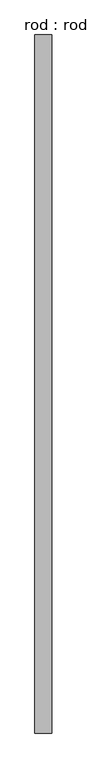
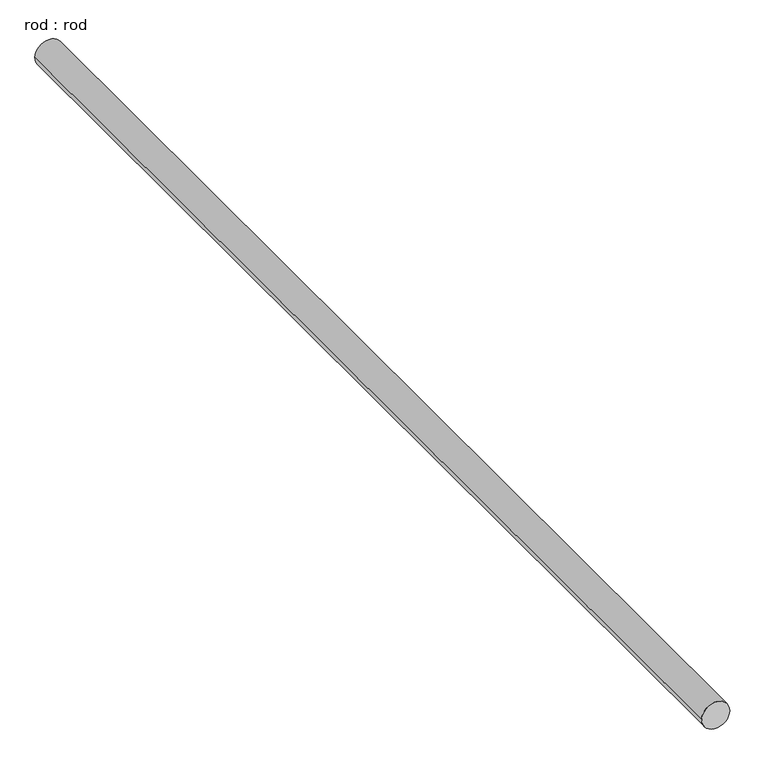
"""IFC4 building model written with IfcOpenShell, lengths in millimetres: proxy geometry, rod : rod."""

from ifc_helpers import new_model, si_unit, point, frame, frame_2d, origin, place, context, project, spatial, circle_curve, trimmed, segment, composite_curve, outline, extrude, source, transform, mapped, element, save


def rod_rod_edea6ea3(model_context):
    return source(origin(), model_context, "Body", "SweptSolid", [
        extrude(outline(composite_curve([segment(trimmed(circle_curve(frame_2d((0.0108462, 0.0)), 200.0), [point((0.0108462, 200.0))], [point((0.0108462, -200.0))], False, "CARTESIAN"), True, "CONTINUOUS"), segment(trimmed(circle_curve(frame_2d((0.0108462, 0.0)), 200.0), [point((0.0108462, -200.0))], [point((0.0108462, 200.0))], False, "CARTESIAN"), True, "CONTINUOUS")], self_intersect=False)), frame((0.0, -4146.8591322, 0.0), z_axis=(0.0, 1.0, 0.0), x_axis=(0.0, 0.0, 1.0)), (0.0, 0.0, 1.0), 16479.1754952),
    ])


if __name__ == "__main__":
    model = new_model("IFC4")
    model_context = context("Model", 3, world=origin())
    ifc_project = project(units=[si_unit("LENGTHUNIT", "METRE", prefix="MILLI")], contexts=[model_context])
    site = spatial("IfcSite", under=ifc_project)
    building = spatial("IfcBuilding", under=site)
    placement = place(None, origin())
    rod_rod_shape = rod_rod_edea6ea3(model_context)
    element("IfcBuildingElementProxy", 1, Name="rod : rod", ObjectType="rod : rod", at=placement, inside=building, context=model_context, shape_type="MappedRepresentation", body=[
        mapped(rod_rod_shape, transform((0.0, 0.0, 0.0), x_axis=(1.0, 0.0, 0.0), y_axis=(0.0, 1.0, 0.0), z_axis=(0.0, 0.0, 1.0))),
    ])
    save(model, "model.ifc")

# Revit data of these elements
# Type "rod : rod"
#   Default Elevation = 0
